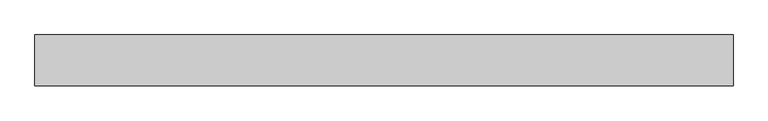
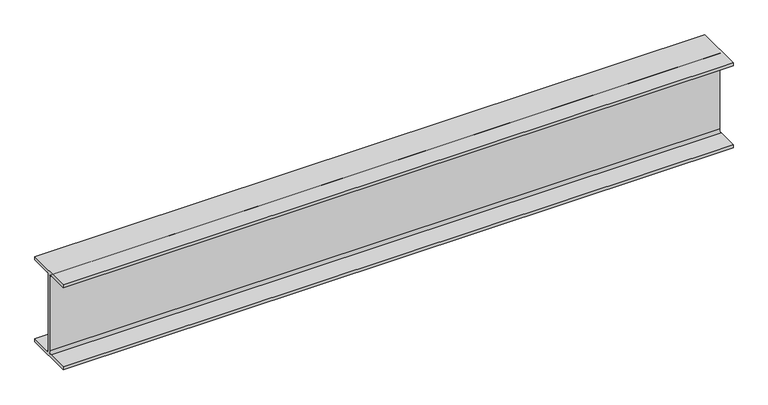
"""IFC4 building model written with IfcOpenShell, lengths in millimetres: beam geometry, Steel Beam_H-KSD3502 : H_SB_ASB_H-200x200x8x12."""

from ifc_helpers import new_model, si_unit, point, frame, frame_2d, origin, place, context, project, spatial, polyline, circle_curve, trimmed, segment, composite_curve, outline, extrude, source, transform, mapped, element, save


def beam_9b741c7f(model_context):
    return source(origin(), model_context, "Body", "SweptSolid", [
        extrude(outline(composite_curve([segment(polyline([(82.5, -141.5), (82.5, -151.7), (-82.5, -151.7), (-82.5, -141.5), (-11.9, -141.5)]), True, "CONTINUOUS"), segment(trimmed(circle_curve(frame_2d((-11.9, -132.6)), 8.9), [point((-11.9, -141.5))], [point((-3.0, -132.6))], True, "CARTESIAN"), True, "CONTINUOUS"), segment(polyline([(-3.0, -132.6), (-3.0, 132.6)]), True, "CONTINUOUS"), segment(trimmed(circle_curve(frame_2d((-11.9, 132.6)), 8.9), [point((-3.0, 132.6))], [point((-11.9, 141.5))], True, "CARTESIAN"), True, "CONTINUOUS"), segment(polyline([(-11.9, 141.5), (-82.5, 141.5), (-82.5, 151.7), (82.5, 151.7), (82.5, 141.5), (11.9, 141.5)]), True, "CONTINUOUS"), segment(trimmed(circle_curve(frame_2d((11.9, 132.6)), 8.9), [point((11.9, 141.5))], [point((3.0, 132.6))], True, "CARTESIAN"), True, "CONTINUOUS"), segment(polyline([(3.0, 132.6), (3.0, -132.6)]), True, "CONTINUOUS"), segment(trimmed(circle_curve(frame_2d((11.9, -132.6)), 8.9), [point((3.0, -132.6))], [point((11.9, -141.5))], True, "CARTESIAN"), True, "CONTINUOUS"), segment(polyline([(11.9, -141.5), (82.5, -141.5)]), True, "CONTINUOUS")], self_intersect=False)), frame((-1289.752068, 0.0, 0.0), z_axis=(1.0, 0.0, 0.0), x_axis=(0.0, 1.0, 0.0)), (0.0, 0.0, 1.0), 2265.6401913),
    ])


if __name__ == "__main__":
    model = new_model("IFC4")
    model_context = context("Model", 3, world=origin())
    ifc_project = project(units=[si_unit("LENGTHUNIT", "METRE", prefix="MILLI")], contexts=[model_context])
    site = spatial("IfcSite", under=ifc_project)
    building = spatial("IfcBuilding", under=site)
    placement = place(None, origin())
    beam_shape = beam_9b741c7f(model_context)
    element("IfcBeam", 1, ObjectType="Steel Beam_H-KSD3502 : H_SB_ASB_H-200x200x8x12", at=placement, inside=building, context=model_context, shape_type="MappedRepresentation", body=[
        mapped(beam_shape, transform((0.0, 0.0, 0.0), x_axis=(1.0, 0.0, 0.0), y_axis=(0.0, 1.0, 0.0), z_axis=(0.0, 0.0, 1.0))),
    ])
    save(model, "model.ifc")

# Revit data of these elements
# Type "Steel Beam_H-KSD3502 : H_SB_ASB_H-200x200x8x12"
#   Width = 20.0 cm
#   Web Thickness = 0.8 cm
#   Web Fillet = 1.3 cm
#   Warping Constant = 141376.0 cm⁶
#   Torsional Moment of Inertia = 26.2485 cm⁴
#   Torsional Modulus = 1.0 cm³
#   Section Area = 63.53 cm²
#   Plastic Modulus weak axis = 244.0 cm³
#   Plastic Modulus strong axis = 525.0 cm³
#   Perimeter = 1.16 m²/m
#   Nominal Weight = 49.90 kgf/m
#   Moment of Inertia weak axis = 1600.00 cm⁴
#   Moment of Inertia strong axis = 4720.00 cm⁴
#   Height = 20.0 cm
#   Flange Thickness = 1.2 cm
#   Elastic Modulus weak axis = 160.0 cm³
#   Elastic Modulus strong axis = 472.0 cm³
#   Centroid Vertical = 10.0 cm
#   Centroid Horizontal = 10.0 cm
#   Length [instance default] = 1.5240 m
#   Structural Material [instance default] = Steel, 45-345
#   Assembly Code = ""
# Element 1 (IfcBeam, "Steel Beam_H-KSD3502 : H_SB_ASB_H-200x200x8x12")
#   Structural Material = none
# Materials
#   "Steel, 45-345": class "Metal", colour RGB 189 187 185, transparency 0, Description = "Steel 345 MPa", Cost = 0
